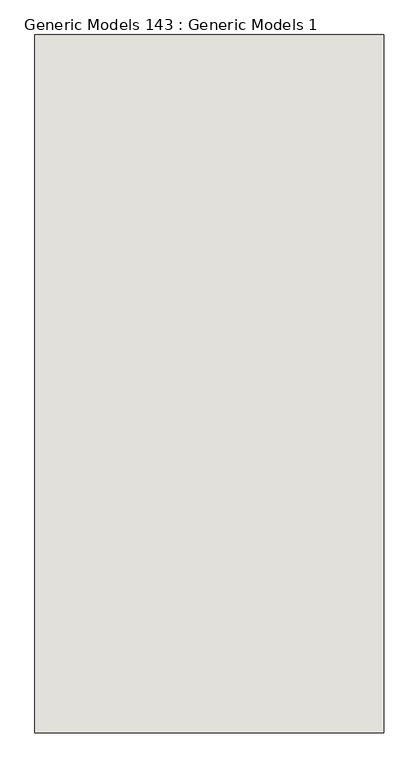
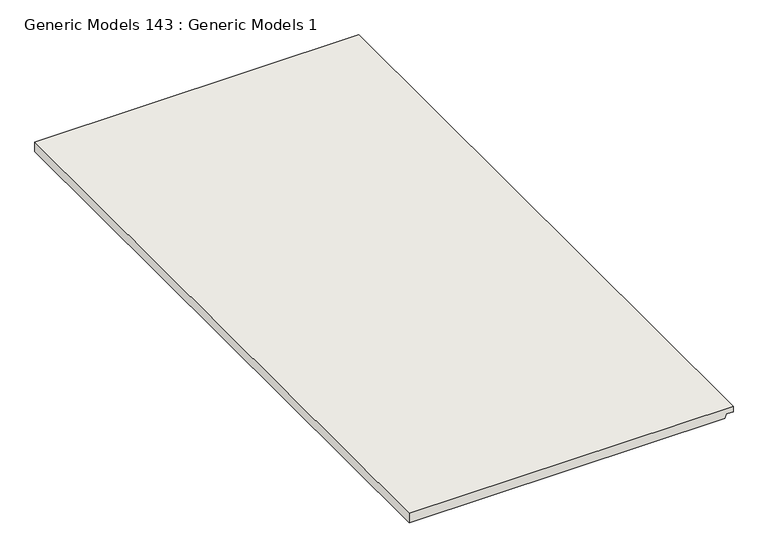
"""IFC4 building model written with IfcOpenShell, lengths in millimetres: wall geometry, Generic Models 143 : Generic Models 1."""

from ifc_helpers import new_model, si_unit, frame, origin, place, context, project, spatial, polyline, outline, extrude, source, transform, mapped, element, save


def generic_models_143_generic_models_1_b888180f(model_context):
    return source(origin(), model_context, "Body", "SweptSolid", [
        extrude(outline(polyline([(1836.9583676, 50897.6548593), (1836.9583676, 50288.0548593), (1817.9083676, 50288.0548593), (1817.9083676, 50882.0658455), (1825.8458676, 50884.9548593), (1825.8458676, 50897.6548593), (1836.9583676, 50897.6548593)])), frame((0.0, 0.0, 0.0), z_axis=(0.0, 1.0, 0.0), x_axis=(0.0, 0.0, 1.0)), (0.0, 0.0, 1.0), 1219.2),
    ])


if __name__ == "__main__":
    model = new_model("IFC4")
    model_context = context("Model", 3, world=origin())
    ifc_project = project(units=[si_unit("LENGTHUNIT", "METRE", prefix="MILLI")], contexts=[model_context])
    site = spatial("IfcSite", under=ifc_project)
    building = spatial("IfcBuilding", under=site)
    placement = place(None, origin())
    generic_models_143_generic_models_1_shape = generic_models_143_generic_models_1_b888180f(model_context)
    element("IfcWall", 1, ObjectType="Generic Models 143 : Generic Models 1", at=placement, inside=building, context=model_context, shape_type="MappedRepresentation", body=[
        mapped(generic_models_143_generic_models_1_shape, transform((0.0, 0.0, 0.0), x_axis=(1.0, 0.0, 0.0), y_axis=(0.0, 1.0, 0.0), z_axis=(0.0, 0.0, 1.0))),
    ])
    save(model, "model.ifc")

# Revit data of these elements
# Element 1 (IfcWall, "Generic Models 143 : Generic Models 1")
#   Materials on its faces: "CEILING AS SCHEDULED"
# Materials
#   "CEILING AS SCHEDULED": class "Generic", colour RGB 255 255 255, transparency 0, Cost = 0
